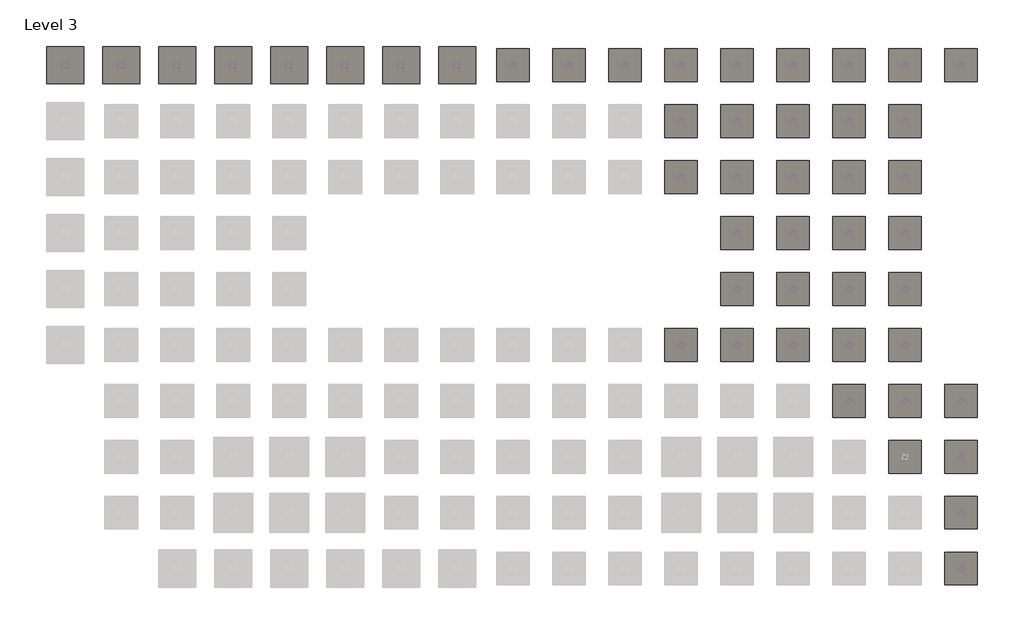
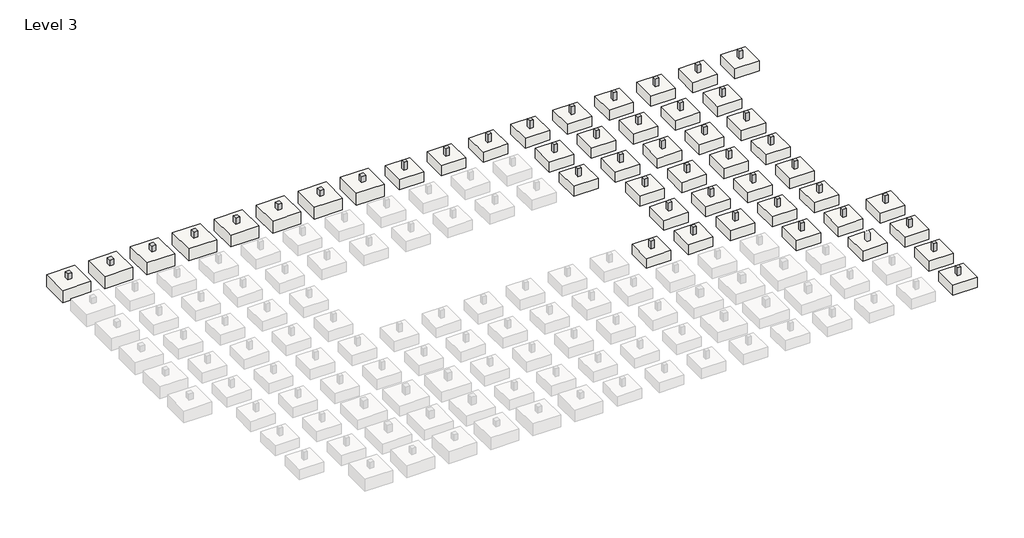
# One storey, part 3 of 3: 47 slabs, 46 columns.
"""IFC4 building model written with IfcOpenShell, lengths in millimetres."""

import ifcopenshell
import ifcopenshell.guid

model = None  # the IFC model being written
_history = None  # IfcOwnerHistory: only IFC2X3 demands one
_inside = {}  # id of a spatial element -> (the spatial element, [elements in it])
_under = {}  # id of a project, library or spatial element -> (it, [spatial elements below it])
_declared = {}  # id of a project -> (the project, [libraries it declares])
_typed = {}  # id of a type object -> (the type object, [elements of that type])
_made_of = {}  # id of a material, layer set ... -> (it, [elements and type objects made of it])


def new_model(schema):
    """Start an empty IFC model of exactly this schema.

    Asked for "IFC4X3", IfcOpenShell would pick the latest addendum, in which some entities
    have other attributes; the version numbers below select the first issue.
    IFC2X3 requires an IfcOwnerHistory on every rooted entity: one is made here for all.
    """
    global model, _history
    if schema == "IFC4X3":
        model = ifcopenshell.file(schema_version=(4, 3, 0, 0))
    else:
        model = ifcopenshell.file(schema=schema)
    _inside.clear()
    _under.clear()
    _declared.clear()
    _typed.clear()
    _made_of.clear()
    _history = None
    if model.schema == "IFC2X3":
        org = make("IfcOrganization", Name="unknown")
        user = make(
            "IfcPersonAndOrganization",
            ThePerson=make("IfcPerson", FamilyName="unknown"),
            TheOrganization=org,
        )
        app = make(
            "IfcApplication",
            ApplicationDeveloper=org,
            Version="unknown",
            ApplicationFullName="unknown",
            ApplicationIdentifier="unknown",
        )
        _history = make(
            "IfcOwnerHistory",
            OwningUser=user,
            OwningApplication=app,
            ChangeAction="ADDED",
            CreationDate=0,
        )
    return model


def make(cls, **values):
    """One entity of the class cls with the attributes given. An attribute that is None is left unset."""
    return model.create_entity(
        cls, **{name: value for name, value in values.items() if value is not None}
    )


def rooted(cls, **values):
    """An entity with a GlobalId (a new one), such as an element, a storey or a relation."""
    return make(cls, GlobalId=ifcopenshell.guid.new(), OwnerHistory=_history, **values)


def si_unit(unit_type, name, prefix=None):
    """IfcSIUnit, for example si_unit("LENGTHUNIT", "METRE", prefix="MILLI")."""
    return make("IfcSIUnit", UnitType=unit_type, Prefix=prefix, Name=name)


def assignment(units):
    """IfcUnitAssignment: the units of a project."""
    return None if units is None else make("IfcUnitAssignment", Units=units)


def point(xyz):
    """IfcCartesianPoint."""
    return None if xyz is None else make("IfcCartesianPoint", Coordinates=xyz)


def direction(xyz):
    """IfcDirection."""
    return None if xyz is None else make("IfcDirection", DirectionRatios=xyz)


def frame(location, z_axis=None, x_axis=None):
    """IfcAxis2Placement3D, a coordinate frame: its origin and axes. An axis left out is left unset."""
    return make(
        "IfcAxis2Placement3D",
        Location=point(location),
        Axis=direction(z_axis),
        RefDirection=direction(x_axis),
    )


def origin():
    """The frame at (0, 0, 0) with its axes left unset."""
    return frame((0.0, 0.0, 0.0))


def origin_with_axes():
    """The frame at (0, 0, 0) with the z axis (0, 0, 1) and the x axis (1, 0, 0) written out."""
    return frame((0.0, 0.0, 0.0), z_axis=(0.0, 0.0, 1.0), x_axis=(1.0, 0.0, 0.0))


def place(relative_to, where):
    """IfcLocalPlacement: puts the frame where relative to a parent placement (None: the world)."""
    return make(
        "IfcLocalPlacement", PlacementRelTo=relative_to, RelativePlacement=where
    )


def context(
    kind, dimensions, precision=None, world=None, true_north=None, identifier=None
):
    """IfcGeometricRepresentationContext, for example the 3D "Model" context."""
    return make(
        "IfcGeometricRepresentationContext",
        ContextIdentifier=identifier,
        ContextType=kind,
        CoordinateSpaceDimension=dimensions,
        Precision=precision,
        WorldCoordinateSystem=world,
        TrueNorth=true_north,
    )


def project(units=None, contexts=None):
    """IfcProject with its units and contexts."""
    return rooted(
        "IfcProject",
        Name="project",
        RepresentationContexts=contexts,
        UnitsInContext=assignment(units),
    )


def spatial(cls, under=None, at=None, **own):
    """A site, building, storey or space (cls), placed at a placement, below another one or the project."""
    s = rooted(cls, ObjectPlacement=at, **own)
    if under is not None:
        _under.setdefault(under.id(), (under, []))[1].append(s)
    return s


def polyline(points):
    """IfcPolyline through the points."""
    return make("IfcPolyline", Points=[point(p) for p in points])


def outline(outer, holes=None, kind="AREA"):
    """IfcArbitraryClosedProfileDef: a profile drawn as a closed curve; with holes, ...WithVoids."""
    if holes is None:
        return make("IfcArbitraryClosedProfileDef", ProfileType=kind, OuterCurve=outer)
    return make(
        "IfcArbitraryProfileDefWithVoids",
        ProfileType=kind,
        OuterCurve=outer,
        InnerCurves=holes,
    )


def extrude(swept, where, along, depth):
    """IfcExtrudedAreaSolid: the profile swept, set in the frame where, extruded along a direction by depth."""
    return make(
        "IfcExtrudedAreaSolid",
        SweptArea=swept,
        Position=where,
        ExtrudedDirection=direction(along),
        Depth=depth,
    )


def shape(context_of_items, identifier, shape_type, items):
    """IfcShapeRepresentation: the items that make up one representation, for example the "Body"."""
    return make(
        "IfcShapeRepresentation",
        ContextOfItems=context_of_items,
        RepresentationIdentifier=identifier,
        RepresentationType=shape_type,
        Items=items,
    )


def source(mapping_origin, context_of_items, identifier, shape_type, items):
    """IfcRepresentationMap: a shape defined once, which mapped items show again and again."""
    return make(
        "IfcRepresentationMap",
        MappingOrigin=mapping_origin,
        MappedRepresentation=shape(context_of_items, identifier, shape_type, items),
    )


def transform(
    local_origin,
    x_axis=None,
    y_axis=None,
    z_axis=None,
    scale=None,
    scale2=None,
    scale3=None,
    uniform=True,
):
    """IfcCartesianTransformationOperator3D, or its non-uniform kind. x_axis, y_axis, z_axis: its Axis1, 2, 3."""
    if uniform:
        return make(
            "IfcCartesianTransformationOperator3D",
            Axis1=direction(x_axis),
            Axis2=direction(y_axis),
            LocalOrigin=point(local_origin),
            Scale=scale,
            Axis3=direction(z_axis),
        )
    return make(
        "IfcCartesianTransformationOperator3DnonUniform",
        Axis1=direction(x_axis),
        Axis2=direction(y_axis),
        LocalOrigin=point(local_origin),
        Scale=scale,
        Axis3=direction(z_axis),
        Scale2=scale2,
        Scale3=scale3,
    )


def mapped(mapping_source, mapping_target):
    """IfcMappedItem: shows the shape of a source again, moved by a transform."""
    return make(
        "IfcMappedItem", MappingSource=mapping_source, MappingTarget=mapping_target
    )


def made_of(thing, what):
    """Note that an element or type object is made of a material, layer set ...; save() writes the relation."""
    if what is not None:
        _made_of.setdefault(what.id(), (what, []))[1].append(thing)
    return thing


def element(
    cls,
    number,
    at=None,
    inside=None,
    cuts=None,
    type_object=None,
    material=None,
    context=None,
    identifier="Body",
    shape_type=None,
    held_by="IfcProductDefinitionShape",
    body=None,
    shapes=None,
    **own,
):
    """One element of the class cls, such as IfcWall. Its Tag is "e" and its number.

    at: its placement. inside: the storey or other place that contains it. cuts: it is an
    opening in that element (IfcRelVoidsElement). A single representation is given by context,
    identifier, shape_type and body (its items); several are given by shapes. held_by: the class
    of the entity that holds the representations. save() writes the other relations.
    """
    e = rooted(cls, Tag="e%d" % number, ObjectPlacement=at, **own)
    if body is not None:
        shapes = [shape(context, identifier, shape_type, body)]
    if shapes is not None:
        e.Representation = make(held_by, Representations=shapes)
    if inside is not None:
        _inside.setdefault(inside.id(), (inside, []))[1].append(e)
    if cuts is not None:
        rooted(
            "IfcRelVoidsElement", RelatingBuildingElement=cuts, RelatedOpeningElement=e
        )
    if type_object is not None:
        _typed.setdefault(type_object.id(), (type_object, []))[1].append(e)
    return made_of(e, material)


def aggregate(whole, parts):
    """IfcRelAggregates: a whole, such as a stair, and the parts it consists of."""
    return rooted("IfcRelAggregates", RelatingObject=whole, RelatedObjects=parts)


def save(model, path):
    """Write the relations noted so far, then the file.

    IfcRelAggregates (storeys below a building ...), IfcRelContainedInSpatialStructure (elements
    in a storey), IfcRelDefinesByType, IfcRelAssociatesMaterial and IfcRelDeclares: one each for
    every whole, place, type object, material and project.
    """
    for whole, parts in _under.values():
        aggregate(whole, parts)
    for where, things in _inside.values():
        rooted(
            "IfcRelContainedInSpatialStructure",
            RelatedElements=things,
            RelatingStructure=where,
        )
    for kind, things in _typed.values():
        rooted("IfcRelDefinesByType", RelatedObjects=things, RelatingType=kind)
    for what, things in _made_of.values():
        rooted("IfcRelAssociatesMaterial", RelatedObjects=things, RelatingMaterial=what)
    for by, libraries in _declared.values():
        rooted("IfcRelDeclares", RelatingContext=by, RelatedDefinitions=libraries)
    model.write(path)


def cl111_concrete_rectangular_column_cl111_500x500_13a722a7(model_context):
    return source(origin(), model_context, "Body", "SweptSolid", [
        extrude(outline(polyline([(250.0, 250.0), (250.0, -250.0), (-250.0, -250.0), (-250.0, 250.0), (250.0, 250.0)])), frame((0.0, 0.0, -1200.0), z_axis=(0.0, 0.0, 1.0), x_axis=(1.0, 0.0, 0.0)), (0.0, 0.0, 1.0), 1200.0),
    ])


def ft111_footing_rectangular_ft111_3500x3500_d0491e67(model_context):
    return source(origin(), model_context, "Body", "SweptSolid", [
        extrude(outline(polyline([(1750.0, 1750.0), (1750.0, -1750.0), (-1750.0, -1750.0), (-1750.0, 1750.0), (1750.0, 1750.0)])), origin_with_axes(), (0.0, 0.0, 1.0), 1500.0),
    ])


model = new_model("IFC4")

# Units and contexts
model_context = context("Model", 3, world=origin())
ifc_project = project(units=[si_unit("LENGTHUNIT", "METRE", prefix="MILLI")], contexts=[model_context])

# Site, building, storey
site = spatial("IfcSite", under=ifc_project)
building = spatial("IfcBuilding", under=site)
storey = spatial("IfcBuildingStorey", under=building, Name="Level 3", Elevation=-2700.0)

# Columns
placement = place(None, origin())
element("IfcColumn", 1, ObjectType="CL111_Concrete-Rectangular-Column : CL111_500x500", at=placement, inside=storey, context=model_context, shape_type="SweptSolid", body=[
    extrude(outline(polyline([(54250.0, 250.0), (54250.0, -250.0), (53750.0, -250.0), (53750.0, 250.0), (54250.0, 250.0)])), frame((0.0, 0.0, -1200.0), z_axis=(0.0, 0.0, 1.0), x_axis=(1.0, 0.0, 0.0)), (0.0, 0.0, 1.0), 1200.0),
])
element("IfcColumn", 2, ObjectType="CL111_Concrete-Rectangular-Column : CL111_500x500", at=placement, inside=storey, context=model_context, shape_type="SweptSolid", body=[
    extrude(outline(polyline([(84250.0, 250.0), (84250.0, -250.0), (83750.0, -250.0), (83750.0, 250.0), (84250.0, 250.0)])), frame((0.0, 0.0, -1200.0), z_axis=(0.0, 0.0, 1.0), x_axis=(1.0, 0.0, 0.0)), (0.0, 0.0, 1.0), 1200.0),
])
element("IfcColumn", 3, ObjectType="CL111_Concrete-Rectangular-Column : CL111_500x500", at=placement, inside=storey, context=model_context, shape_type="SweptSolid", body=[
    extrude(outline(polyline([(48250.0, 250.0), (48250.0, -250.0), (47750.0, -250.0), (47750.0, 250.0), (48250.0, 250.0)])), frame((0.0, 0.0, -1200.0), z_axis=(0.0, 0.0, 1.0), x_axis=(1.0, 0.0, 0.0)), (0.0, 0.0, 1.0), 1200.0),
])
element("IfcColumn", 4, ObjectType="CL111_Concrete-Rectangular-Column : CL111_500x500", at=placement, inside=storey, context=model_context, shape_type="SweptSolid", body=[
    extrude(outline(polyline([(90250.0, 250.0), (90250.0, -250.0), (89750.0, -250.0), (89750.0, 250.0), (90250.0, 250.0)])), frame((0.0, 0.0, -1200.0), z_axis=(0.0, 0.0, 1.0), x_axis=(1.0, 0.0, 0.0)), (0.0, 0.0, 1.0), 1200.0),
])
element("IfcColumn", 5, ObjectType="CL111_Concrete-Rectangular-Column : CL111_500x500", at=placement, inside=storey, context=model_context, shape_type="SweptSolid", body=[
    extrude(outline(polyline([(72250.0, 250.0), (72250.0, -250.0), (71750.0, -250.0), (71750.0, 250.0), (72250.0, 250.0)])), frame((0.0, 0.0, -1200.0), z_axis=(0.0, 0.0, 1.0), x_axis=(1.0, 0.0, 0.0)), (0.0, 0.0, 1.0), 1200.0),
])
element("IfcColumn", 6, ObjectType="CL111_Concrete-Rectangular-Column : CL111_500x500", at=placement, inside=storey, context=model_context, shape_type="SweptSolid", body=[
    extrude(outline(polyline([(78250.0, 250.0), (78250.0, -250.0), (77750.0, -250.0), (77750.0, 250.0), (78250.0, 250.0)])), frame((0.0, 0.0, -1200.0), z_axis=(0.0, 0.0, 1.0), x_axis=(1.0, 0.0, 0.0)), (0.0, 0.0, 1.0), 1200.0),
])
element("IfcColumn", 7, ObjectType="CL111_Concrete-Rectangular-Column : CL111_500x500", at=placement, inside=storey, context=model_context, shape_type="SweptSolid", body=[
    extrude(outline(polyline([(60250.0, 250.0), (60250.0, -250.0), (59750.0, -250.0), (59750.0, 250.0), (60250.0, 250.0)])), frame((0.0, 0.0, -1200.0), z_axis=(0.0, 0.0, 1.0), x_axis=(1.0, 0.0, 0.0)), (0.0, 0.0, 1.0), 1200.0),
])
element("IfcColumn", 8, ObjectType="CL111_Concrete-Rectangular-Column : CL111_500x500", at=placement, inside=storey, context=model_context, shape_type="SweptSolid", body=[
    extrude(outline(polyline([(66250.0, 250.0), (66250.0, -250.0), (65750.0, -250.0), (65750.0, 250.0), (66250.0, 250.0)])), frame((0.0, 0.0, -1200.0), z_axis=(0.0, 0.0, 1.0), x_axis=(1.0, 0.0, 0.0)), (0.0, 0.0, 1.0), 1200.0),
])
element("IfcColumn", 9, ObjectType="CL111_Concrete-Rectangular-Column : CL111_500x500", at=placement, inside=storey, context=model_context, shape_type="SweptSolid", body=[
    extrude(outline(polyline([(96250.0, -35750.0), (96250.0, -36250.0), (95750.0, -36250.0), (95750.0, -35750.0), (96250.0, -35750.0)])), frame((0.0, 0.0, -1200.0), z_axis=(0.0, 0.0, 1.0), x_axis=(1.0, 0.0, 0.0)), (0.0, 0.0, 1.0), 1200.0),
])
element("IfcColumn", 10, ObjectType="CL111_Concrete-Rectangular-Column : CL111_500x500", at=placement, inside=storey, context=model_context, shape_type="SweptSolid", body=[
    extrude(outline(polyline([(96250.0, 250.0), (96250.0, -250.0), (95750.0, -250.0), (95750.0, 250.0), (96250.0, 250.0)])), frame((0.0, 0.0, -1200.0), z_axis=(0.0, 0.0, 1.0), x_axis=(1.0, 0.0, 0.0)), (0.0, 0.0, 1.0), 1200.0),
])
element("IfcColumn", 11, ObjectType="CL111_Concrete-Rectangular-Column : CL111_500x500", at=placement, inside=storey, context=model_context, shape_type="SweptSolid", body=[
    extrude(outline(polyline([(96250.0, -47750.0), (96250.0, -48250.0), (95750.0, -48250.0), (95750.0, -47750.0), (96250.0, -47750.0)])), frame((0.0, 0.0, -1200.0), z_axis=(0.0, 0.0, 1.0), x_axis=(1.0, 0.0, 0.0)), (0.0, 0.0, 1.0), 1200.0),
])
element("IfcColumn", 12, ObjectType="CL111_Concrete-Rectangular-Column : CL111_500x500", at=placement, inside=storey, context=model_context, shape_type="SweptSolid", body=[
    extrude(outline(polyline([(96250.0, -41750.0), (96250.0, -42250.0), (95750.0, -42250.0), (95750.0, -41750.0), (96250.0, -41750.0)])), frame((0.0, 0.0, -1200.0), z_axis=(0.0, 0.0, 1.0), x_axis=(1.0, 0.0, 0.0)), (0.0, 0.0, 1.0), 1200.0),
])
element("IfcColumn", 13, ObjectType="CL111_Concrete-Rectangular-Column : CL111_500x500", at=placement, inside=storey, context=model_context, shape_type="SweptSolid", body=[
    extrude(outline(polyline([(96250.0, -53750.0), (96250.0, -54250.0), (95750.0, -54250.0), (95750.0, -53750.0), (96250.0, -53750.0)])), frame((0.0, 0.0, -1200.0), z_axis=(0.0, 0.0, 1.0), x_axis=(1.0, 0.0, 0.0)), (0.0, 0.0, 1.0), 1200.0),
])
cl111_concrete_rectangular_column_cl111_500x500_shape = cl111_concrete_rectangular_column_cl111_500x500_13a722a7(model_context)
element("IfcColumn", 14, ObjectType="CL111_Concrete-Rectangular-Column : CL111_500x500", at=placement, inside=storey, context=model_context, shape_type="MappedRepresentation", body=[
    mapped(cl111_concrete_rectangular_column_cl111_500x500_shape, transform((84000.0, -24000.0, 0.0), x_axis=(1.0, 0.0, 0.0), y_axis=(0.0, 1.0, 0.0), z_axis=(0.0, 0.0, 1.0))),
])
element("IfcColumn", 15, ObjectType="CL111_Concrete-Rectangular-Column : CL111_500x500", at=placement, inside=storey, context=model_context, shape_type="MappedRepresentation", body=[
    mapped(cl111_concrete_rectangular_column_cl111_500x500_shape, transform((84000.0, -36000.0, 0.0), x_axis=(1.0, 0.0, 0.0), y_axis=(0.0, 1.0, 0.0), z_axis=(0.0, 0.0, 1.0))),
])
element("IfcColumn", 16, ObjectType="CL111_Concrete-Rectangular-Column : CL111_500x500", at=placement, inside=storey, context=model_context, shape_type="MappedRepresentation", body=[
    mapped(cl111_concrete_rectangular_column_cl111_500x500_shape, transform((84000.0, -18000.0, 0.0), x_axis=(1.0, 0.0, 0.0), y_axis=(0.0, 1.0, 0.0), z_axis=(0.0, 0.0, 1.0))),
])
element("IfcColumn", 17, ObjectType="CL111_Concrete-Rectangular-Column : CL111_500x500", at=placement, inside=storey, context=model_context, shape_type="MappedRepresentation", body=[
    mapped(cl111_concrete_rectangular_column_cl111_500x500_shape, transform((84000.0, -30000.0, 0.0), x_axis=(1.0, 0.0, 0.0), y_axis=(0.0, 1.0, 0.0), z_axis=(0.0, 0.0, 1.0))),
])
element("IfcColumn", 18, ObjectType="CL111_Concrete-Rectangular-Column : CL111_500x500", at=placement, inside=storey, context=model_context, shape_type="MappedRepresentation", body=[
    mapped(cl111_concrete_rectangular_column_cl111_500x500_shape, transform((84000.0, -12000.0, 0.0), x_axis=(1.0, 0.0, 0.0), y_axis=(0.0, 1.0, 0.0), z_axis=(0.0, 0.0, 1.0))),
])
element("IfcColumn", 19, ObjectType="CL111_Concrete-Rectangular-Column : CL111_500x500", at=placement, inside=storey, context=model_context, shape_type="MappedRepresentation", body=[
    mapped(cl111_concrete_rectangular_column_cl111_500x500_shape, transform((84000.0, -6000.0, 0.0), x_axis=(1.0, 0.0, 0.0), y_axis=(0.0, 1.0, 0.0), z_axis=(0.0, 0.0, 1.0))),
])
element("IfcColumn", 20, ObjectType="CL111_Concrete-Rectangular-Column : CL111_500x500", at=placement, inside=storey, context=model_context, shape_type="MappedRepresentation", body=[
    mapped(cl111_concrete_rectangular_column_cl111_500x500_shape, transform((90000.0, -24000.0, 0.0), x_axis=(1.0, 0.0, 0.0), y_axis=(0.0, 1.0, 0.0), z_axis=(0.0, 0.0, 1.0))),
])
element("IfcColumn", 21, ObjectType="CL111_Concrete-Rectangular-Column : CL111_500x500", at=placement, inside=storey, context=model_context, shape_type="MappedRepresentation", body=[
    mapped(cl111_concrete_rectangular_column_cl111_500x500_shape, transform((90000.0, -36000.0, 0.0), x_axis=(1.0, 0.0, 0.0), y_axis=(0.0, 1.0, 0.0), z_axis=(0.0, 0.0, 1.0))),
])
element("IfcColumn", 22, ObjectType="CL111_Concrete-Rectangular-Column : CL111_500x500", at=placement, inside=storey, context=model_context, shape_type="MappedRepresentation", body=[
    mapped(cl111_concrete_rectangular_column_cl111_500x500_shape, transform((90000.0, -18000.0, 0.0), x_axis=(1.0, 0.0, 0.0), y_axis=(0.0, 1.0, 0.0), z_axis=(0.0, 0.0, 1.0))),
])
element("IfcColumn", 23, ObjectType="CL111_Concrete-Rectangular-Column : CL111_500x500", at=placement, inside=storey, context=model_context, shape_type="MappedRepresentation", body=[
    mapped(cl111_concrete_rectangular_column_cl111_500x500_shape, transform((90000.0, -30000.0, 0.0), x_axis=(1.0, 0.0, 0.0), y_axis=(0.0, 1.0, 0.0), z_axis=(0.0, 0.0, 1.0))),
])
element("IfcColumn", 24, ObjectType="CL111_Concrete-Rectangular-Column : CL111_500x500", at=placement, inside=storey, context=model_context, shape_type="MappedRepresentation", body=[
    mapped(cl111_concrete_rectangular_column_cl111_500x500_shape, transform((90000.0, -12000.0, 0.0), x_axis=(1.0, 0.0, 0.0), y_axis=(0.0, 1.0, 0.0), z_axis=(0.0, 0.0, 1.0))),
])
element("IfcColumn", 25, ObjectType="CL111_Concrete-Rectangular-Column : CL111_500x500", at=placement, inside=storey, context=model_context, shape_type="MappedRepresentation", body=[
    mapped(cl111_concrete_rectangular_column_cl111_500x500_shape, transform((90000.0, -6000.0, 0.0), x_axis=(1.0, 0.0, 0.0), y_axis=(0.0, 1.0, 0.0), z_axis=(0.0, 0.0, 1.0))),
])
element("IfcColumn", 26, ObjectType="CL111_Concrete-Rectangular-Column : CL111_500x500", at=placement, inside=storey, context=model_context, shape_type="MappedRepresentation", body=[
    mapped(cl111_concrete_rectangular_column_cl111_500x500_shape, transform((72000.0, -24000.0, 0.0), x_axis=(1.0, 0.0, 0.0), y_axis=(0.0, 1.0, 0.0), z_axis=(0.0, 0.0, 1.0))),
])
element("IfcColumn", 27, ObjectType="CL111_Concrete-Rectangular-Column : CL111_500x500", at=placement, inside=storey, context=model_context, shape_type="MappedRepresentation", body=[
    mapped(cl111_concrete_rectangular_column_cl111_500x500_shape, transform((72000.0, -18000.0, 0.0), x_axis=(1.0, 0.0, 0.0), y_axis=(0.0, 1.0, 0.0), z_axis=(0.0, 0.0, 1.0))),
])
element("IfcColumn", 28, ObjectType="CL111_Concrete-Rectangular-Column : CL111_500x500", at=placement, inside=storey, context=model_context, shape_type="MappedRepresentation", body=[
    mapped(cl111_concrete_rectangular_column_cl111_500x500_shape, transform((72000.0, -30000.0, 0.0), x_axis=(1.0, 0.0, 0.0), y_axis=(0.0, 1.0, 0.0), z_axis=(0.0, 0.0, 1.0))),
])
element("IfcColumn", 29, ObjectType="CL111_Concrete-Rectangular-Column : CL111_500x500", at=placement, inside=storey, context=model_context, shape_type="MappedRepresentation", body=[
    mapped(cl111_concrete_rectangular_column_cl111_500x500_shape, transform((72000.0, -12000.0, 0.0), x_axis=(1.0, 0.0, 0.0), y_axis=(0.0, 1.0, 0.0), z_axis=(0.0, 0.0, 1.0))),
])
element("IfcColumn", 30, ObjectType="CL111_Concrete-Rectangular-Column : CL111_500x500", at=placement, inside=storey, context=model_context, shape_type="MappedRepresentation", body=[
    mapped(cl111_concrete_rectangular_column_cl111_500x500_shape, transform((72000.0, -6000.0, 0.0), x_axis=(1.0, 0.0, 0.0), y_axis=(0.0, 1.0, 0.0), z_axis=(0.0, 0.0, 1.0))),
])
element("IfcColumn", 31, ObjectType="CL111_Concrete-Rectangular-Column : CL111_500x500", at=placement, inside=storey, context=model_context, shape_type="MappedRepresentation", body=[
    mapped(cl111_concrete_rectangular_column_cl111_500x500_shape, transform((78000.0, -24000.0, 0.0), x_axis=(1.0, 0.0, 0.0), y_axis=(0.0, 1.0, 0.0), z_axis=(0.0, 0.0, 1.0))),
])
element("IfcColumn", 32, ObjectType="CL111_Concrete-Rectangular-Column : CL111_500x500", at=placement, inside=storey, context=model_context, shape_type="MappedRepresentation", body=[
    mapped(cl111_concrete_rectangular_column_cl111_500x500_shape, transform((78000.0, -18000.0, 0.0), x_axis=(1.0, 0.0, 0.0), y_axis=(0.0, 1.0, 0.0), z_axis=(0.0, 0.0, 1.0))),
])
element("IfcColumn", 33, ObjectType="CL111_Concrete-Rectangular-Column : CL111_500x500", at=placement, inside=storey, context=model_context, shape_type="MappedRepresentation", body=[
    mapped(cl111_concrete_rectangular_column_cl111_500x500_shape, transform((78000.0, -30000.0, 0.0), x_axis=(1.0, 0.0, 0.0), y_axis=(0.0, 1.0, 0.0), z_axis=(0.0, 0.0, 1.0))),
])
element("IfcColumn", 34, ObjectType="CL111_Concrete-Rectangular-Column : CL111_500x500", at=placement, inside=storey, context=model_context, shape_type="MappedRepresentation", body=[
    mapped(cl111_concrete_rectangular_column_cl111_500x500_shape, transform((78000.0, -12000.0, 0.0), x_axis=(1.0, 0.0, 0.0), y_axis=(0.0, 1.0, 0.0), z_axis=(0.0, 0.0, 1.0))),
])
element("IfcColumn", 35, ObjectType="CL111_Concrete-Rectangular-Column : CL111_500x500", at=placement, inside=storey, context=model_context, shape_type="MappedRepresentation", body=[
    mapped(cl111_concrete_rectangular_column_cl111_500x500_shape, transform((78000.0, -6000.0, 0.0), x_axis=(1.0, 0.0, 0.0), y_axis=(0.0, 1.0, 0.0), z_axis=(0.0, 0.0, 1.0))),
])
element("IfcColumn", 36, ObjectType="CL111_Concrete-Rectangular-Column : CL111_500x500", at=placement, inside=storey, context=model_context, shape_type="MappedRepresentation", body=[
    mapped(cl111_concrete_rectangular_column_cl111_500x500_shape, transform((66000.0, -30000.0, 0.0), x_axis=(1.0, 0.0, 0.0), y_axis=(0.0, 1.0, 0.0), z_axis=(0.0, 0.0, 1.0))),
])
element("IfcColumn", 37, ObjectType="CL111_Concrete-Rectangular-Column : CL111_500x500", at=placement, inside=storey, context=model_context, shape_type="MappedRepresentation", body=[
    mapped(cl111_concrete_rectangular_column_cl111_500x500_shape, transform((66000.0, -12000.0, 0.0), x_axis=(1.0, 0.0, 0.0), y_axis=(0.0, 1.0, 0.0), z_axis=(0.0, 0.0, 1.0))),
])
element("IfcColumn", 38, ObjectType="CL111_Concrete-Rectangular-Column : CL111_500x500", at=placement, inside=storey, context=model_context, shape_type="MappedRepresentation", body=[
    mapped(cl111_concrete_rectangular_column_cl111_500x500_shape, transform((66000.0, -6000.0, 0.0), x_axis=(1.0, 0.0, 0.0), y_axis=(0.0, 1.0, 0.0), z_axis=(0.0, 0.0, 1.0))),
])
element("IfcColumn", 39, ObjectType="CL111_Concrete-Rectangular-Column : CL111_600x600", at=placement, inside=storey, context=model_context, shape_type="SweptSolid", body=[
    extrude(outline(polyline([(18300.0, 300.0), (18300.0, -300.0), (17700.0, -300.0), (17700.0, 300.0), (18300.0, 300.0)])), frame((0.0, 0.0, -900.0), z_axis=(0.0, 0.0, 1.0), x_axis=(1.0, 0.0, 0.0)), (0.0, 0.0, 1.0), 900.0),
])
element("IfcColumn", 40, ObjectType="CL111_Concrete-Rectangular-Column : CL111_600x600", at=placement, inside=storey, context=model_context, shape_type="SweptSolid", body=[
    extrude(outline(polyline([(24300.0, 300.0), (24300.0, -300.0), (23700.0, -300.0), (23700.0, 300.0), (24300.0, 300.0)])), frame((0.0, 0.0, -900.0), z_axis=(0.0, 0.0, 1.0), x_axis=(1.0, 0.0, 0.0)), (0.0, 0.0, 1.0), 900.0),
])
element("IfcColumn", 41, ObjectType="CL111_Concrete-Rectangular-Column : CL111_600x600", at=placement, inside=storey, context=model_context, shape_type="SweptSolid", body=[
    extrude(outline(polyline([(30300.0, 300.0), (30300.0, -300.0), (29700.0, -300.0), (29700.0, 300.0), (30300.0, 300.0)])), frame((0.0, 0.0, -900.0), z_axis=(0.0, 0.0, 1.0), x_axis=(1.0, 0.0, 0.0)), (0.0, 0.0, 1.0), 900.0),
])
element("IfcColumn", 42, ObjectType="CL111_Concrete-Rectangular-Column : CL111_600x600", at=placement, inside=storey, context=model_context, shape_type="SweptSolid", body=[
    extrude(outline(polyline([(36300.0, 300.0), (36300.0, -300.0), (35700.0, -300.0), (35700.0, 300.0), (36300.0, 300.0)])), frame((0.0, 0.0, -900.0), z_axis=(0.0, 0.0, 1.0), x_axis=(1.0, 0.0, 0.0)), (0.0, 0.0, 1.0), 900.0),
])
element("IfcColumn", 43, ObjectType="CL111_Concrete-Rectangular-Column : CL111_600x600", at=placement, inside=storey, context=model_context, shape_type="SweptSolid", body=[
    extrude(outline(polyline([(300.0, 300.0), (300.0, -300.0), (-300.0, -300.0), (-300.0, 300.0), (300.0, 300.0)])), frame((0.0, 0.0, -900.0), z_axis=(0.0, 0.0, 1.0), x_axis=(1.0, 0.0, 0.0)), (0.0, 0.0, 1.0), 900.0),
])
element("IfcColumn", 44, ObjectType="CL111_Concrete-Rectangular-Column : CL111_600x600", at=placement, inside=storey, context=model_context, shape_type="SweptSolid", body=[
    extrude(outline(polyline([(6300.0, 300.0), (6300.0, -300.0), (5700.0, -300.0), (5700.0, 300.0), (6300.0, 300.0)])), frame((0.0, 0.0, -900.0), z_axis=(0.0, 0.0, 1.0), x_axis=(1.0, 0.0, 0.0)), (0.0, 0.0, 1.0), 900.0),
])
element("IfcColumn", 45, ObjectType="CL111_Concrete-Rectangular-Column : CL111_600x600", at=placement, inside=storey, context=model_context, shape_type="SweptSolid", body=[
    extrude(outline(polyline([(12300.0, 300.0), (12300.0, -300.0), (11700.0, -300.0), (11700.0, 300.0), (12300.0, 300.0)])), frame((0.0, 0.0, -900.0), z_axis=(0.0, 0.0, 1.0), x_axis=(1.0, 0.0, 0.0)), (0.0, 0.0, 1.0), 900.0),
])
element("IfcColumn", 46, ObjectType="CL111_Concrete-Rectangular-Column : CL111_600x600", at=placement, inside=storey, context=model_context, shape_type="SweptSolid", body=[
    extrude(outline(polyline([(42300.0, 300.0), (42300.0, -300.0), (41700.0, -300.0), (41700.0, 300.0), (42300.0, 300.0)])), frame((0.0, 0.0, -900.0), z_axis=(0.0, 0.0, 1.0), x_axis=(1.0, 0.0, 0.0)), (0.0, 0.0, 1.0), 900.0),
])

# Slabs
element("IfcSlab", 47, ObjectType="FT111_Footing-Rectangular : FT111_3500x3500", at=placement, inside=storey, context=model_context, shape_type="SweptSolid", body=[
    extrude(outline(polyline([(55750.0, 1750.0), (55750.0, -1750.0), (52250.0, -1750.0), (52250.0, 1750.0), (55750.0, 1750.0)])), frame((0.0, 0.0, -2700.0), z_axis=(0.0, 0.0, 1.0), x_axis=(1.0, 0.0, 0.0)), (0.0, 0.0, 1.0), 1500.0),
])
element("IfcSlab", 48, ObjectType="FT111_Footing-Rectangular : FT111_3500x3500", at=placement, inside=storey, context=model_context, shape_type="SweptSolid", body=[
    extrude(outline(polyline([(85750.0, 1750.0), (85750.0, -1750.0), (82250.0, -1750.0), (82250.0, 1750.0), (85750.0, 1750.0)])), frame((0.0, 0.0, -2700.0), z_axis=(0.0, 0.0, 1.0), x_axis=(1.0, 0.0, 0.0)), (0.0, 0.0, 1.0), 1500.0),
])
element("IfcSlab", 49, ObjectType="FT111_Footing-Rectangular : FT111_3500x3500", at=placement, inside=storey, context=model_context, shape_type="SweptSolid", body=[
    extrude(outline(polyline([(49750.0, 1750.0), (49750.0, -1750.0), (46250.0, -1750.0), (46250.0, 1750.0), (49750.0, 1750.0)])), frame((0.0, 0.0, -2700.0), z_axis=(0.0, 0.0, 1.0), x_axis=(1.0, 0.0, 0.0)), (0.0, 0.0, 1.0), 1500.0),
])
element("IfcSlab", 50, ObjectType="FT111_Footing-Rectangular : FT111_3500x3500", at=placement, inside=storey, context=model_context, shape_type="SweptSolid", body=[
    extrude(outline(polyline([(91750.0, 1750.0), (91750.0, -1750.0), (88250.0, -1750.0), (88250.0, 1750.0), (91750.0, 1750.0)])), frame((0.0, 0.0, -2700.0), z_axis=(0.0, 0.0, 1.0), x_axis=(1.0, 0.0, 0.0)), (0.0, 0.0, 1.0), 1500.0),
])
element("IfcSlab", 51, ObjectType="FT111_Footing-Rectangular : FT111_3500x3500", at=placement, inside=storey, context=model_context, shape_type="SweptSolid", body=[
    extrude(outline(polyline([(73750.0, 1750.0), (73750.0, -1750.0), (70250.0, -1750.0), (70250.0, 1750.0), (73750.0, 1750.0)])), frame((0.0, 0.0, -2700.0), z_axis=(0.0, 0.0, 1.0), x_axis=(1.0, 0.0, 0.0)), (0.0, 0.0, 1.0), 1500.0),
])
element("IfcSlab", 52, ObjectType="FT111_Footing-Rectangular : FT111_3500x3500", at=placement, inside=storey, context=model_context, shape_type="SweptSolid", body=[
    extrude(outline(polyline([(79750.0, 1750.0), (79750.0, -1750.0), (76250.0, -1750.0), (76250.0, 1750.0), (79750.0, 1750.0)])), frame((0.0, 0.0, -2700.0), z_axis=(0.0, 0.0, 1.0), x_axis=(1.0, 0.0, 0.0)), (0.0, 0.0, 1.0), 1500.0),
])
element("IfcSlab", 53, ObjectType="FT111_Footing-Rectangular : FT111_3500x3500", at=placement, inside=storey, context=model_context, shape_type="SweptSolid", body=[
    extrude(outline(polyline([(61750.0, 1750.0), (61750.0, -1750.0), (58250.0, -1750.0), (58250.0, 1750.0), (61750.0, 1750.0)])), frame((0.0, 0.0, -2700.0), z_axis=(0.0, 0.0, 1.0), x_axis=(1.0, 0.0, 0.0)), (0.0, 0.0, 1.0), 1500.0),
])
element("IfcSlab", 54, ObjectType="FT111_Footing-Rectangular : FT111_3500x3500", at=placement, inside=storey, context=model_context, shape_type="SweptSolid", body=[
    extrude(outline(polyline([(67750.0, 1750.0), (67750.0, -1750.0), (64250.0, -1750.0), (64250.0, 1750.0), (67750.0, 1750.0)])), frame((0.0, 0.0, -2700.0), z_axis=(0.0, 0.0, 1.0), x_axis=(1.0, 0.0, 0.0)), (0.0, 0.0, 1.0), 1500.0),
])
element("IfcSlab", 55, ObjectType="FT111_Footing-Rectangular : FT111_3500x3500", at=placement, inside=storey, context=model_context, shape_type="SweptSolid", body=[
    extrude(outline(polyline([(97750.0, -34250.0), (97750.0, -37750.0), (94250.0, -37750.0), (94250.0, -34250.0), (97750.0, -34250.0)])), frame((0.0, 0.0, -2700.0), z_axis=(0.0, 0.0, 1.0), x_axis=(1.0, 0.0, 0.0)), (0.0, 0.0, 1.0), 1500.0),
])
element("IfcSlab", 56, ObjectType="FT111_Footing-Rectangular : FT111_3500x3500", at=placement, inside=storey, context=model_context, shape_type="SweptSolid", body=[
    extrude(outline(polyline([(97750.0, 1750.0), (97750.0, -1750.0), (94250.0, -1750.0), (94250.0, 1750.0), (97750.0, 1750.0)])), frame((0.0, 0.0, -2700.0), z_axis=(0.0, 0.0, 1.0), x_axis=(1.0, 0.0, 0.0)), (0.0, 0.0, 1.0), 1500.0),
])
element("IfcSlab", 57, ObjectType="FT111_Footing-Rectangular : FT111_3500x3500", at=placement, inside=storey, context=model_context, shape_type="SweptSolid", body=[
    extrude(outline(polyline([(97750.0, -46250.0), (97750.0, -49750.0), (94250.0, -49750.0), (94250.0, -46250.0), (97750.0, -46250.0)])), frame((0.0, 0.0, -2700.0), z_axis=(0.0, 0.0, 1.0), x_axis=(1.0, 0.0, 0.0)), (0.0, 0.0, 1.0), 1500.0),
])
element("IfcSlab", 58, ObjectType="FT111_Footing-Rectangular : FT111_3500x3500", at=placement, inside=storey, context=model_context, shape_type="SweptSolid", body=[
    extrude(outline(polyline([(97750.0, -40250.0), (97750.0, -43750.0), (94250.0, -43750.0), (94250.0, -40250.0), (97750.0, -40250.0)])), frame((0.0, 0.0, -2700.0), z_axis=(0.0, 0.0, 1.0), x_axis=(1.0, 0.0, 0.0)), (0.0, 0.0, 1.0), 1500.0),
])
element("IfcSlab", 59, ObjectType="FT111_Footing-Rectangular : FT111_3500x3500", at=placement, inside=storey, context=model_context, shape_type="SweptSolid", body=[
    extrude(outline(polyline([(97750.0, -52250.0), (97750.0, -55750.0), (94250.0, -55750.0), (94250.0, -52250.0), (97750.0, -52250.0)])), frame((0.0, 0.0, -2700.0), z_axis=(0.0, 0.0, 1.0), x_axis=(1.0, 0.0, 0.0)), (0.0, 0.0, 1.0), 1500.0),
])
ft111_footing_rectangular_ft111_3500x3500_shape = ft111_footing_rectangular_ft111_3500x3500_d0491e67(model_context)
element("IfcSlab", 60, ObjectType="FT111_Footing-Rectangular : FT111_3500x3500", at=placement, inside=storey, context=model_context, shape_type="MappedRepresentation", body=[
    mapped(ft111_footing_rectangular_ft111_3500x3500_shape, transform((84000.0, -24000.0, -2700.0), x_axis=(1.0, 0.0, 0.0), y_axis=(0.0, 1.0, 0.0), z_axis=(0.0, 0.0, 1.0))),
])
element("IfcSlab", 61, ObjectType="FT111_Footing-Rectangular : FT111_3500x3500", at=placement, inside=storey, context=model_context, shape_type="MappedRepresentation", body=[
    mapped(ft111_footing_rectangular_ft111_3500x3500_shape, transform((84000.0, -36000.0, -2700.0), x_axis=(1.0, 0.0, 0.0), y_axis=(0.0, 1.0, 0.0), z_axis=(0.0, 0.0, 1.0))),
])
element("IfcSlab", 62, ObjectType="FT111_Footing-Rectangular : FT111_3500x3500", at=placement, inside=storey, context=model_context, shape_type="MappedRepresentation", body=[
    mapped(ft111_footing_rectangular_ft111_3500x3500_shape, transform((84000.0, -18000.0, -2700.0), x_axis=(1.0, 0.0, 0.0), y_axis=(0.0, 1.0, 0.0), z_axis=(0.0, 0.0, 1.0))),
])
element("IfcSlab", 63, ObjectType="FT111_Footing-Rectangular : FT111_3500x3500", at=placement, inside=storey, context=model_context, shape_type="MappedRepresentation", body=[
    mapped(ft111_footing_rectangular_ft111_3500x3500_shape, transform((84000.0, -30000.0, -2700.0), x_axis=(1.0, 0.0, 0.0), y_axis=(0.0, 1.0, 0.0), z_axis=(0.0, 0.0, 1.0))),
])
element("IfcSlab", 64, ObjectType="FT111_Footing-Rectangular : FT111_3500x3500", at=placement, inside=storey, context=model_context, shape_type="MappedRepresentation", body=[
    mapped(ft111_footing_rectangular_ft111_3500x3500_shape, transform((84000.0, -12000.0, -2700.0), x_axis=(1.0, 0.0, 0.0), y_axis=(0.0, 1.0, 0.0), z_axis=(0.0, 0.0, 1.0))),
])
element("IfcSlab", 65, ObjectType="FT111_Footing-Rectangular : FT111_3500x3500", at=placement, inside=storey, context=model_context, shape_type="MappedRepresentation", body=[
    mapped(ft111_footing_rectangular_ft111_3500x3500_shape, transform((84000.0, -6000.0, -2700.0), x_axis=(1.0, 0.0, 0.0), y_axis=(0.0, 1.0, 0.0), z_axis=(0.0, 0.0, 1.0))),
])
element("IfcSlab", 66, ObjectType="FT111_Footing-Rectangular : FT111_3500x3500", at=placement, inside=storey, context=model_context, shape_type="MappedRepresentation", body=[
    mapped(ft111_footing_rectangular_ft111_3500x3500_shape, transform((90000.0, -24000.0, -2700.0), x_axis=(1.0, 0.0, 0.0), y_axis=(0.0, 1.0, 0.0), z_axis=(0.0, 0.0, 1.0))),
])
element("IfcSlab", 67, ObjectType="FT111_Footing-Rectangular : FT111_3500x3500", at=placement, inside=storey, context=model_context, shape_type="MappedRepresentation", body=[
    mapped(ft111_footing_rectangular_ft111_3500x3500_shape, transform((90000.0, -36000.0, -2700.0), x_axis=(1.0, 0.0, 0.0), y_axis=(0.0, 1.0, 0.0), z_axis=(0.0, 0.0, 1.0))),
])
element("IfcSlab", 68, ObjectType="FT111_Footing-Rectangular : FT111_3500x3500", at=placement, inside=storey, context=model_context, shape_type="MappedRepresentation", body=[
    mapped(ft111_footing_rectangular_ft111_3500x3500_shape, transform((90000.0, -18000.0, -2700.0), x_axis=(1.0, 0.0, 0.0), y_axis=(0.0, 1.0, 0.0), z_axis=(0.0, 0.0, 1.0))),
])
element("IfcSlab", 69, ObjectType="FT111_Footing-Rectangular : FT111_3500x3500", at=placement, inside=storey, context=model_context, shape_type="MappedRepresentation", body=[
    mapped(ft111_footing_rectangular_ft111_3500x3500_shape, transform((90000.0, -30000.0, -2700.0), x_axis=(1.0, 0.0, 0.0), y_axis=(0.0, 1.0, 0.0), z_axis=(0.0, 0.0, 1.0))),
])
element("IfcSlab", 70, ObjectType="FT111_Footing-Rectangular : FT111_3500x3500", at=placement, inside=storey, context=model_context, shape_type="MappedRepresentation", body=[
    mapped(ft111_footing_rectangular_ft111_3500x3500_shape, transform((90000.0, -12000.0, -2700.0), x_axis=(1.0, 0.0, 0.0), y_axis=(0.0, 1.0, 0.0), z_axis=(0.0, 0.0, 1.0))),
])
element("IfcSlab", 71, ObjectType="FT111_Footing-Rectangular : FT111_3500x3500", at=placement, inside=storey, context=model_context, shape_type="MappedRepresentation", body=[
    mapped(ft111_footing_rectangular_ft111_3500x3500_shape, transform((90000.0, -6000.0, -2700.0), x_axis=(1.0, 0.0, 0.0), y_axis=(0.0, 1.0, 0.0), z_axis=(0.0, 0.0, 1.0))),
])
element("IfcSlab", 72, ObjectType="FT111_Footing-Rectangular : FT111_3500x3500", at=placement, inside=storey, context=model_context, shape_type="MappedRepresentation", body=[
    mapped(ft111_footing_rectangular_ft111_3500x3500_shape, transform((90000.0, -42000.0, -2700.0), x_axis=(1.0, 0.0, 0.0), y_axis=(0.0, 1.0, 0.0), z_axis=(0.0, 0.0, 1.0))),
])
element("IfcSlab", 73, ObjectType="FT111_Footing-Rectangular : FT111_3500x3500", at=placement, inside=storey, context=model_context, shape_type="MappedRepresentation", body=[
    mapped(ft111_footing_rectangular_ft111_3500x3500_shape, transform((72000.0, -24000.0, -2700.0), x_axis=(1.0, 0.0, 0.0), y_axis=(0.0, 1.0, 0.0), z_axis=(0.0, 0.0, 1.0))),
])
element("IfcSlab", 74, ObjectType="FT111_Footing-Rectangular : FT111_3500x3500", at=placement, inside=storey, context=model_context, shape_type="MappedRepresentation", body=[
    mapped(ft111_footing_rectangular_ft111_3500x3500_shape, transform((72000.0, -18000.0, -2700.0), x_axis=(1.0, 0.0, 0.0), y_axis=(0.0, 1.0, 0.0), z_axis=(0.0, 0.0, 1.0))),
])
element("IfcSlab", 75, ObjectType="FT111_Footing-Rectangular : FT111_3500x3500", at=placement, inside=storey, context=model_context, shape_type="MappedRepresentation", body=[
    mapped(ft111_footing_rectangular_ft111_3500x3500_shape, transform((72000.0, -30000.0, -2700.0), x_axis=(1.0, 0.0, 0.0), y_axis=(0.0, 1.0, 0.0), z_axis=(0.0, 0.0, 1.0))),
])
element("IfcSlab", 76, ObjectType="FT111_Footing-Rectangular : FT111_3500x3500", at=placement, inside=storey, context=model_context, shape_type="MappedRepresentation", body=[
    mapped(ft111_footing_rectangular_ft111_3500x3500_shape, transform((72000.0, -12000.0, -2700.0), x_axis=(1.0, 0.0, 0.0), y_axis=(0.0, 1.0, 0.0), z_axis=(0.0, 0.0, 1.0))),
])
element("IfcSlab", 77, ObjectType="FT111_Footing-Rectangular : FT111_3500x3500", at=placement, inside=storey, context=model_context, shape_type="MappedRepresentation", body=[
    mapped(ft111_footing_rectangular_ft111_3500x3500_shape, transform((72000.0, -6000.0, -2700.0), x_axis=(1.0, 0.0, 0.0), y_axis=(0.0, 1.0, 0.0), z_axis=(0.0, 0.0, 1.0))),
])
element("IfcSlab", 78, ObjectType="FT111_Footing-Rectangular : FT111_3500x3500", at=placement, inside=storey, context=model_context, shape_type="MappedRepresentation", body=[
    mapped(ft111_footing_rectangular_ft111_3500x3500_shape, transform((78000.0, -24000.0, -2700.0), x_axis=(1.0, 0.0, 0.0), y_axis=(0.0, 1.0, 0.0), z_axis=(0.0, 0.0, 1.0))),
])
element("IfcSlab", 79, ObjectType="FT111_Footing-Rectangular : FT111_3500x3500", at=placement, inside=storey, context=model_context, shape_type="MappedRepresentation", body=[
    mapped(ft111_footing_rectangular_ft111_3500x3500_shape, transform((78000.0, -18000.0, -2700.0), x_axis=(1.0, 0.0, 0.0), y_axis=(0.0, 1.0, 0.0), z_axis=(0.0, 0.0, 1.0))),
])
element("IfcSlab", 80, ObjectType="FT111_Footing-Rectangular : FT111_3500x3500", at=placement, inside=storey, context=model_context, shape_type="MappedRepresentation", body=[
    mapped(ft111_footing_rectangular_ft111_3500x3500_shape, transform((78000.0, -30000.0, -2700.0), x_axis=(1.0, 0.0, 0.0), y_axis=(0.0, 1.0, 0.0), z_axis=(0.0, 0.0, 1.0))),
])
element("IfcSlab", 81, ObjectType="FT111_Footing-Rectangular : FT111_3500x3500", at=placement, inside=storey, context=model_context, shape_type="MappedRepresentation", body=[
    mapped(ft111_footing_rectangular_ft111_3500x3500_shape, transform((78000.0, -12000.0, -2700.0), x_axis=(1.0, 0.0, 0.0), y_axis=(0.0, 1.0, 0.0), z_axis=(0.0, 0.0, 1.0))),
])
element("IfcSlab", 82, ObjectType="FT111_Footing-Rectangular : FT111_3500x3500", at=placement, inside=storey, context=model_context, shape_type="MappedRepresentation", body=[
    mapped(ft111_footing_rectangular_ft111_3500x3500_shape, transform((78000.0, -6000.0, -2700.0), x_axis=(1.0, 0.0, 0.0), y_axis=(0.0, 1.0, 0.0), z_axis=(0.0, 0.0, 1.0))),
])
element("IfcSlab", 83, ObjectType="FT111_Footing-Rectangular : FT111_3500x3500", at=placement, inside=storey, context=model_context, shape_type="MappedRepresentation", body=[
    mapped(ft111_footing_rectangular_ft111_3500x3500_shape, transform((66000.0, -30000.0, -2700.0), x_axis=(1.0, 0.0, 0.0), y_axis=(0.0, 1.0, 0.0), z_axis=(0.0, 0.0, 1.0))),
])
element("IfcSlab", 84, ObjectType="FT111_Footing-Rectangular : FT111_3500x3500", at=placement, inside=storey, context=model_context, shape_type="MappedRepresentation", body=[
    mapped(ft111_footing_rectangular_ft111_3500x3500_shape, transform((66000.0, -12000.0, -2700.0), x_axis=(1.0, 0.0, 0.0), y_axis=(0.0, 1.0, 0.0), z_axis=(0.0, 0.0, 1.0))),
])
element("IfcSlab", 85, ObjectType="FT111_Footing-Rectangular : FT111_3500x3500", at=placement, inside=storey, context=model_context, shape_type="MappedRepresentation", body=[
    mapped(ft111_footing_rectangular_ft111_3500x3500_shape, transform((66000.0, -6000.0, -2700.0), x_axis=(1.0, 0.0, 0.0), y_axis=(0.0, 1.0, 0.0), z_axis=(0.0, 0.0, 1.0))),
])
element("IfcSlab", 86, ObjectType="FT111_Footing-Rectangular : FT111_4000x4000", at=placement, inside=storey, context=model_context, shape_type="SweptSolid", body=[
    extrude(outline(polyline([(20000.0, 2000.0), (20000.0, -2000.0), (16000.0, -2000.0), (16000.0, 2000.0), (20000.0, 2000.0)])), frame((0.0, 0.0, -2700.0), z_axis=(0.0, 0.0, 1.0), x_axis=(1.0, 0.0, 0.0)), (0.0, 0.0, 1.0), 1800.0),
])
element("IfcSlab", 87, ObjectType="FT111_Footing-Rectangular : FT111_4000x4000", at=placement, inside=storey, context=model_context, shape_type="SweptSolid", body=[
    extrude(outline(polyline([(26000.0, 2000.0), (26000.0, -2000.0), (22000.0, -2000.0), (22000.0, 2000.0), (26000.0, 2000.0)])), frame((0.0, 0.0, -2700.0), z_axis=(0.0, 0.0, 1.0), x_axis=(1.0, 0.0, 0.0)), (0.0, 0.0, 1.0), 1800.0),
])
element("IfcSlab", 88, ObjectType="FT111_Footing-Rectangular : FT111_4000x4000", at=placement, inside=storey, context=model_context, shape_type="SweptSolid", body=[
    extrude(outline(polyline([(32000.0, 2000.0), (32000.0, -2000.0), (28000.0, -2000.0), (28000.0, 2000.0), (32000.0, 2000.0)])), frame((0.0, 0.0, -2700.0), z_axis=(0.0, 0.0, 1.0), x_axis=(1.0, 0.0, 0.0)), (0.0, 0.0, 1.0), 1800.0),
])
element("IfcSlab", 89, ObjectType="FT111_Footing-Rectangular : FT111_4000x4000", at=placement, inside=storey, context=model_context, shape_type="SweptSolid", body=[
    extrude(outline(polyline([(38000.0, 2000.0), (38000.0, -2000.0), (34000.0, -2000.0), (34000.0, 2000.0), (38000.0, 2000.0)])), frame((0.0, 0.0, -2700.0), z_axis=(0.0, 0.0, 1.0), x_axis=(1.0, 0.0, 0.0)), (0.0, 0.0, 1.0), 1800.0),
])
element("IfcSlab", 90, ObjectType="FT111_Footing-Rectangular : FT111_4000x4000", at=placement, inside=storey, context=model_context, shape_type="SweptSolid", body=[
    extrude(outline(polyline([(2000.0, 2000.0), (2000.0, -2000.0), (-2000.0, -2000.0), (-2000.0, 2000.0), (2000.0, 2000.0)])), frame((0.0, 0.0, -2700.0), z_axis=(0.0, 0.0, 1.0), x_axis=(1.0, 0.0, 0.0)), (0.0, 0.0, 1.0), 1800.0),
])
element("IfcSlab", 91, ObjectType="FT111_Footing-Rectangular : FT111_4000x4000", at=placement, inside=storey, context=model_context, shape_type="SweptSolid", body=[
    extrude(outline(polyline([(8000.0, 2000.0), (8000.0, -2000.0), (4000.0, -2000.0), (4000.0, 2000.0), (8000.0, 2000.0)])), frame((0.0, 0.0, -2700.0), z_axis=(0.0, 0.0, 1.0), x_axis=(1.0, 0.0, 0.0)), (0.0, 0.0, 1.0), 1800.0),
])
element("IfcSlab", 92, ObjectType="FT111_Footing-Rectangular : FT111_4000x4000", at=placement, inside=storey, context=model_context, shape_type="SweptSolid", body=[
    extrude(outline(polyline([(14000.0, 2000.0), (14000.0, -2000.0), (10000.0, -2000.0), (10000.0, 2000.0), (14000.0, 2000.0)])), frame((0.0, 0.0, -2700.0), z_axis=(0.0, 0.0, 1.0), x_axis=(1.0, 0.0, 0.0)), (0.0, 0.0, 1.0), 1800.0),
])
element("IfcSlab", 93, ObjectType="FT111_Footing-Rectangular : FT111_4000x4000", at=placement, inside=storey, context=model_context, shape_type="SweptSolid", body=[
    extrude(outline(polyline([(44000.0, 2000.0), (44000.0, -2000.0), (40000.0, -2000.0), (40000.0, 2000.0), (44000.0, 2000.0)])), frame((0.0, 0.0, -2700.0), z_axis=(0.0, 0.0, 1.0), x_axis=(1.0, 0.0, 0.0)), (0.0, 0.0, 1.0), 1800.0),
])

save(model, "model.ifc")

# Revit data of these elements
# Type "CL111_Concrete-Rectangular-Column : CL111_500x500"
#   Assembly Code = "B10"
#   b = 500 mm
#   h = 500 mm
#   Structural Material [instance default] = Concrete, Cast-in-Place gray
# Type "CL111_Concrete-Rectangular-Column : CL111_600x600"
#   Assembly Code = "B10"
#   b = 600 mm
#   h = 600 mm
#   Structural Material [instance default] = Concrete, Cast-in-Place gray
# Type "FT111_Footing-Rectangular : FT111_3500x3500"
#   Assembly Code = "A1010100"
#   Width = 3500 mm
#   Length = 3500 mm
#   Foundation Thickness = 1500 mm
#   Structural Material [instance default] = Concrete, Cast-in-Place gray
# Type "FT111_Footing-Rectangular : FT111_4000x4000"
#   Assembly Code = "A1010100"
#   Width = 4000 mm
#   Length = 4000 mm
#   Foundation Thickness = 1800 mm
#   Structural Material [instance default] = Concrete, Cast-in-Place gray
# Elements 1, 2, 3, 4, 5, 6, 7, 8, 9, 10, 11, 12, 13, 14, 15, 16, 17, 18, 19, 20, 21, 22, 23, 24, 25, 26, 27, 28, 29, 30, 31, 32, 33, 34, 35, 36, 37, 38 (IfcColumn, "CL111_Concrete-Rectangular-Column : CL111_500x500")
#   Structural Material = Concrete, Cast-in-Place gray
#   Phase Created = New Construction
#   Materials on its faces: "Concrete, Cast-in-Place gray"
# Elements 39, 40, 41, 42, 43, 44, 45, 46 (IfcColumn, "CL111_Concrete-Rectangular-Column : CL111_600x600")
#   Structural Material = Concrete, Cast-in-Place gray
#   Phase Created = New Construction
#   Materials on its faces: "Concrete, Cast-in-Place gray"
# Elements 47, 48, 49, 50, 51, 52, 53, 54, 55, 56, 57, 58, 59, 60, 61, 62, 63, 64, 65, 66, 67, 68, 69, 70, 71, 72, 73, 74, 75, 76, 77, 78, 79, 80, 81, 82, 83, 84, 85 (IfcSlab, "FT111_Footing-Rectangular : FT111_3500x3500")
#   Structural Material = Concrete, Cast-in-Place gray
#   Phase Created = New Construction
#   Materials on its faces: "Concrete, Cast-in-Place gray"
# Elements 86, 87, 88, 89, 90, 91, 92, 93 (IfcSlab, "FT111_Footing-Rectangular : FT111_4000x4000")
#   Structural Material = Concrete, Cast-in-Place gray
#   Phase Created = New Construction
#   Materials on its faces: "Concrete, Cast-in-Place gray"
# Materials
#   "Concrete, Cast-in-Place gray": class "Concrete", colour RGB 192 192 192, transparency 0, Description = "Cast-in-place concrete", Cost = 0
